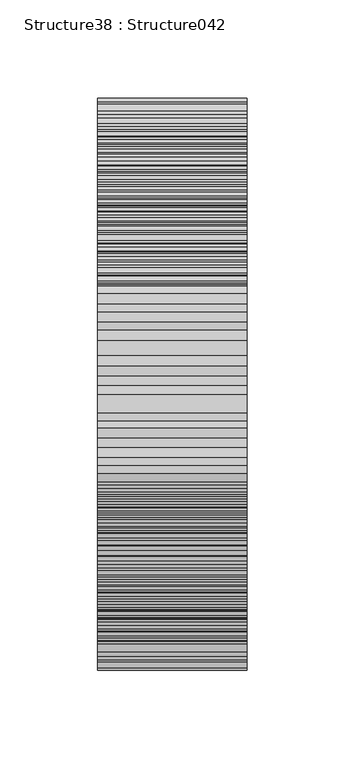
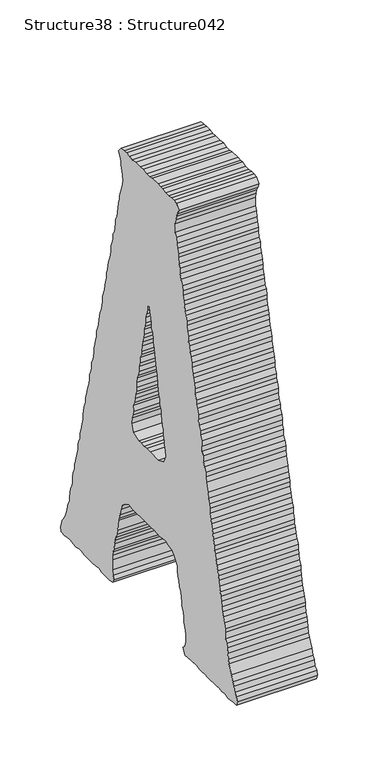
"""IFC4 building model written with IfcOpenShell, lengths in millimetres: proxy geometry, Structure38 : Structure042."""

from ifc_helpers import new_model, si_unit, frame, origin, place, context, project, spatial, polyline, outline, extrude, source, transform, mapped, element, save


def structure38_structure042_37ec2216(model_context):
    return source(origin(), model_context, "Body", "SweptSolid", [
        extrude(outline(polyline([(257160.5137356, 3818.8310229), (257162.8548535, 3824.1149855), (257163.4565802, 3828.2163546), (257164.0358425, 3833.4730389), (257165.7736291, 3838.1761347), (257166.3753558, 3841.6741725), (257168.1356069, 3846.9757858), (257168.1356069, 3851.6612309), (257169.8974627, 3856.9179152), (257171.0784516, 3861.0192843), (257172.236976, 3866.3032469), (257173.3955005, 3870.4030114), (257173.9747627, 3875.0772243), (257175.7366184, 3878.5784713), (257176.3383451, 3884.4609514), (257176.3383451, 3888.5623205), (257177.519334, 3893.822214), (257179.2795852, 3896.763454), (257180.4156451, 3902.6314927), (257181.5966341, 3906.1487857), (257182.777623, 3910.8310217), (257182.777623, 3915.5068392), (257183.9602165, 3919.6066036), (257185.7204676, 3924.8905662), (257187.4582543, 3929.5904528), (257187.4582543, 3934.8503464), (257189.2185054, 3938.3499888), (257190.3994943, 3944.235678), (257190.3994943, 3947.7337158), (257192.1613501, 3952.435207), (257192.7406123, 3957.1190475), (257193.9216012, 3962.3757319), (257195.6593879, 3966.5043792), (257195.6593879, 3974.7055128), (257194.5008634, 3979.3781211), (257193.342339, 3984.0635662), (257191.5596234, 3987.5792547), (257189.2185054, 3992.2614906), (257193.342339, 3996.9645864), (257197.419639, 3997.5486624), (257201.5434725, 3997.5486624), (257206.8033661, 3996.390138), (257211.4823928, 3996.390138), (257216.7647508, 3997.5486624), (257220.285253, 3996.9645864), (257224.3866221, 3997.5486624), (257233.7462802, 3997.5486624), (257238.4493759, 3996.390138), (257243.1300073, 3996.390138), (257248.3882962, 3997.5486624), (257253.6931186, 3996.9645864), (257261.2925255, 3996.9645864), (257266.5748835, 3996.390138), (257270.6521836, 3997.5486624), (257275.957006, 3997.5486624), (257280.0359107, 3996.9645864), (257285.2941996, 3996.390138), (257288.8387709, 3991.6806238), (257286.4751885, 3987.5792547), (257285.2941996, 3983.4794902), (257284.7374018, 3979.9621971), (257283.5564129, 3974.7055128), (257281.7961618, 3965.8930249), (257282.9771507, 3961.794865), (257284.1581396, 3956.5349715), (257287.657782, 3947.1496398), (257287.657782, 3944.235678), (257288.8387709, 3938.9517154), (257289.9972954, 3934.2758979), (257290.599022, 3928.9919353), (257291.780011, 3924.2888396), (257294.0970598, 3919.6066036), (257294.0970598, 3916.0909152), (257294.6779267, 3910.8310217), (257295.8589156, 3906.1487857), (257298.2208934, 3902.6314927), (257298.2208934, 3897.3475301), (257299.9586801, 3892.6636896), (257301.1172045, 3888.5623205), (257301.1172045, 3883.8881076), (257302.299798, 3878.5784713), (257304.0600492, 3873.9203044), (257305.8203003, 3869.8189354), (257306.422027, 3866.3032469), (257307.0012892, 3861.0192843), (257308.7390759, 3856.9179152), (257308.7390759, 3851.6612309), (257310.5009316, 3846.9757858), (257311.1026583, 3842.8583706), (257312.2611827, 3837.6000817), (257315.1799583, 3829.374879), (257315.1799583, 3824.1149855), (257316.3609472, 3820.015221), (257317.5435407, 3815.3313805), (257319.8830541, 3810.0474179), (257320.4847808, 3806.5317294), (257321.6433052, 3801.8462843), (257322.2450319, 3797.1463977), (257323.9828186, 3791.8865042), (257325.1654121, 3788.3611881), (257325.1654121, 3783.0868532), (257326.9256632, 3777.8285642), (257327.5049254, 3774.3032481), (257329.2651766, 3769.0176809), (257329.8669033, 3764.3611187), (257330.423701, 3759.6596275), (257331.6046899, 3756.1423345), (257333.3665457, 3751.4424479), (257333.9458079, 3745.6000829), (257335.1267968, 3740.9162424), (257336.8870479, 3737.9750024), (257336.8870479, 3732.7167134), (257338.0455724, 3727.4311462), (257339.8074281, 3723.3313817), (257340.988417, 3718.0554422), (257342.1469415, 3714.5301261), (257343.3279304, 3710.4560353), (257343.3279304, 3705.7545441), (257345.6449793, 3699.8881101), (257346.8275728, 3695.2122926), (257347.4292995, 3691.0868544), (257347.4292995, 3686.4030139), (257348.5878239, 3682.8857208), (257350.348075, 3677.0449605), (257350.9498017, 3673.5276674), (257352.6875884, 3668.8261762), (257352.6875884, 3663.5598643), (257355.0287064, 3659.4584952), (257356.2096953, 3655.3587307), (257356.2096953, 3650.6845178), (257357.3906842, 3645.4262289), (257359.1509353, 3640.114988), (257360.3094598, 3636.0408972), (257361.4695888, 3632.5155811), (257362.0713155, 3627.2396415), (257363.8315666, 3622.555801), (257365.0125555, 3617.2718384), (257365.0125555, 3612.5976255), (257365.5918178, 3608.4705827), (257367.9313311, 3604.3964919), (257369.0914602, 3599.1125293), (257370.2724491, 3594.4286888), (257370.2724491, 3590.3289243), (257372.0327002, 3586.2115092), (257374.9514758, 3576.2693797), (257376.7133315, 3572.1423369), (257378.4735826, 3568.6426945), (257381.9940849, 3563.366755), (257383.1526094, 3560.441561), (257384.9144651, 3555.1848766), (257383.7334762, 3551.0658569), (257377.8943204, 3550.4833855), (257374.394678, 3551.0658569), (257369.0914602, 3551.6675836), (257364.4108288, 3550.4833855), (257359.1509353, 3550.4833855), (257354.4494441, 3551.6675836), (257350.348075, 3551.6675836), (257345.6449793, 3551.0658569), (257341.5676792, 3551.0658569), (257335.706059, 3550.4833855), (257331.6046899, 3550.4833855), (257326.9256632, 3551.0658569), (257321.6433052, 3551.6675836), (257317.5435407, 3550.4833855), (257304.0600492, 3550.4833855), (257298.8001556, 3551.6675836), (257296.4381778, 3555.7416744), (257298.2208934, 3559.2669905), (257299.3794178, 3563.9412034), (257299.3794178, 3573.9266571), (257299.3794178, 3578.6104977), (257298.2208934, 3582.7102621), (257296.4381778, 3586.2115092), (257295.8589156, 3592.0955938), (257294.6779267, 3596.1953583), (257292.9160709, 3600.2967274), (257291.780011, 3604.3964919), (257290.599022, 3609.0723094), (257289.4180331, 3619.6145609), (257288.2370442, 3622.555801), (257286.4751885, 3627.2396415), (257285.2941996, 3633.0980525), (257282.3978885, 3638.9580681), (257278.2740549, 3642.4833842), (257271.8331725, 3645.9830266), (257267.1541458, 3644.8245022), (257257.7720233, 3644.8245022), (257251.9104031, 3645.4262289), (257239.6303648, 3645.4262289), (257234.3255424, 3644.8245022), (257230.2482424, 3645.9830266), (257225.5451466, 3645.4262289), (257220.8661199, 3644.8245022), (257216.7647508, 3645.4262289), (257210.9031306, 3645.9830266), (257207.3826283, 3644.8245022), (257200.3624836, 3643.0578326), (257196.8403768, 3639.5405396), (257192.1613501, 3633.0980525), (257192.1613501, 3627.8397636), (257190.9803611, 3622.555801), (257189.2185054, 3619.6145609), (257188.6392432, 3613.772196), (257186.2997298, 3610.2292293), (257185.1187409, 3604.9709403), (257184.5394787, 3601.4536473), (257184.5394787, 3596.7698067), (257182.1983607, 3592.0955938), (257181.5966341, 3587.3860796), (257181.0173718, 3582.7102621), (257179.2795852, 3578.6104977), (257177.519334, 3572.7440636), (257178.0985963, 3565.1254015), (257179.8588474, 3559.2669905), (257182.777623, 3556.3417965), (257179.2795852, 3550.4833855), (257173.9747627, 3551.0658569), (257169.295736, 3551.6675836), (257159.9344734, 3551.6675836), (257155.2554467, 3551.0658569), (257150.5523509, 3551.0658569), (257146.4525864, 3551.6675836), (257142.3287528, 3551.0658569), (257136.4895971, 3551.0658569), (257132.9915593, 3551.6675836), (257127.1299391, 3551.0658569), (257123.6078322, 3551.6675836), (257118.9288055, 3550.4833855), (257113.623983, 3551.6675836), (257108.3640895, 3550.4833855), (257104.264325, 3551.0658569), (257099.5612292, 3551.6675836), (257094.904667, 3551.6675836), (257093.1203468, 3556.3417965), (257094.3029403, 3560.441561), (257097.2441803, 3563.366755), (257098.4027048, 3568.6426945), (257100.1629559, 3572.1423369), (257102.5040739, 3577.4535778), (257106.6038383, 3586.2115092), (257107.7848273, 3589.7544759), (257108.3640895, 3595.5872132), (257109.546683, 3600.2967274), (257110.7052074, 3604.3964919), (257112.4654586, 3607.8961343), (257113.0447208, 3613.772196), (257113.0447208, 3617.2718384), (257114.2257097, 3622.555801), (257115.9859608, 3627.8397636), (257117.7478166, 3631.915459), (257118.9288055, 3636.0408972), (257119.5080677, 3641.2991861), (257120.0648655, 3645.9830266), (257120.6665921, 3650.1004418), (257123.0061055, 3654.1841602), (257123.6078322, 3660.0682449), (257124.188699, 3664.1423357), (257124.7679612, 3668.8261762), (257126.5282124, 3672.9435914), (257128.2884635, 3677.6274319), (257129.4469879, 3682.8857208), (257130.6279769, 3685.8285655), (257130.6279769, 3690.512406), (257132.3898326, 3695.786741), (257132.9915593, 3701.0723082), (257134.1500837, 3704.5879966), (257135.8878704, 3709.2718371), (257136.4895971, 3713.3555556), (257138.2498482, 3718.6571688), (257138.2498482, 3723.3313817), (257139.4324417, 3727.4311462), (257140.5909662, 3732.1149867), (257141.7719551, 3737.400554), (257144.1114684, 3746.1745313), (257145.2699929, 3750.8583719), (257145.2699929, 3755.559863), (257147.0318486, 3759.6596275), (257148.7920997, 3763.759392), (257148.7920997, 3769.6274306), (257151.1316131, 3773.11905), (257151.1316131, 3777.8285642), (257151.7108753, 3783.0868532), (257154.0744577, 3787.7867397), (257154.0744577, 3791.8865042), (257156.4139711, 3795.960595), (257157.0156978, 3801.8462843), (257157.0156978, 3805.9476534), (257159.3327467, 3811.2043377), (257160.5137356, 3814.7296538), (257160.5137356, 3818.8310229)]), holes=[polyline([(257223.2056332, 3720.4158154), (257236.6891248, 3720.4158154), (257241.9474137, 3720.9726131), (257247.2297717, 3719.8140887), (257251.3311408, 3720.9726131), (257255.4309053, 3720.4158154), (257264.2113011, 3723.3313817), (257267.1541458, 3730.9323932), (257265.9731569, 3736.7988273), (257264.8130278, 3740.9162424), (257263.6320389, 3744.9999608), (257264.2113011, 3750.8583719), (257261.8942522, 3754.9854146), (257261.2925255, 3759.6596275), (257260.7132633, 3763.759392), (257258.9530122, 3767.8607611), (257258.3512855, 3772.5606477), (257258.3512855, 3777.2444882), (257257.7720233, 3782.5027771), (257256.0101675, 3786.0280932), (257254.8516431, 3790.7039107), (257254.8516431, 3795.4037973), (257252.5121297, 3800.6717138), (257252.5121297, 3805.9476534), (257250.7518786, 3810.0474179), (257250.1501519, 3813.5743386), (257249.5692851, 3819.4150989), (257248.3882962, 3824.1149855), (257247.2297717, 3828.790803), (257246.6505095, 3832.8921721), (257246.6505095, 3837.6000817), (257244.3109962, 3842.2758992), (257243.7092695, 3846.3772683), (257243.7092695, 3851.6612309), (257241.9474137, 3856.3161885), (257240.7664248, 3860.4432313), (257240.7664248, 3864.5446004), (257239.0286382, 3865.1190488), (257237.8701137, 3860.4432313), (257236.0873981, 3855.7353217), (257235.5081359, 3851.0595042), (257235.5081359, 3845.8012153), (257233.1670179, 3842.2758992), (257232.5652913, 3836.9919366), (257232.5652913, 3833.4730389), (257230.2482424, 3828.790803), (257229.6465157, 3822.932392), (257229.0672535, 3818.8310229), (257227.8862645, 3814.7296538), (257227.3053977, 3810.0474179), (257225.5451466, 3804.7730829), (257224.9434199, 3795.4037973), (257223.8073599, 3790.7039107), (257223.2056332, 3786.0280932), (257221.4453821, 3783.0868532), (257221.4453821, 3777.8285642), (257219.1042641, 3773.11905), (257219.1042641, 3768.4432325), (257217.9232752, 3764.3611187), (257217.344013, 3759.0595054), (257215.6062263, 3755.559863), (257215.6062263, 3750.3015741), (257213.8235107, 3744.9999608), (257213.8235107, 3741.5003184), (257212.6633817, 3736.7988273), (257211.4823928, 3730.9323932), (257215.0044997, 3723.9154578), (257223.2056332, 3720.4158154)])]), frame((-38594.2176606, 0.0, 0.0), z_axis=(1.0, 0.0, 0.0), x_axis=(0.0, 1.0, 0.0)), (0.0, 0.0, 1.0), 76.2),
    ])


if __name__ == "__main__":
    model = new_model("IFC4")
    model_context = context("Model", 3, world=origin())
    ifc_project = project(units=[si_unit("LENGTHUNIT", "METRE", prefix="MILLI")], contexts=[model_context])
    site = spatial("IfcSite", under=ifc_project)
    building = spatial("IfcBuilding", under=site)
    placement = place(None, origin())
    structure38_structure042_shape = structure38_structure042_37ec2216(model_context)
    element("IfcBuildingElementProxy", 1, Name="Structure38 : Structure042", ObjectType="Structure38 : Structure042", at=placement, inside=building, context=model_context, shape_type="MappedRepresentation", body=[
        mapped(structure38_structure042_shape, transform((0.0, 0.0, 0.0), x_axis=(1.0, 0.0, 0.0), y_axis=(0.0, 1.0, 0.0), z_axis=(0.0, 0.0, 1.0))),
    ])
    save(model, "model.ifc")

# Revit data of these elements
# Type "Structure38 : Structure042"
#   NameOverride = "Structure042"
# Element 1 (IfcBuildingElementProxy, "Structure38 : Structure042")
#   Materials on its faces: "BRUSHED ALUM. LETTERING"
# Materials
#   "BRUSHED ALUM. LETTERING": class "Unassigned", colour RGB 169 181 186, transparency 0, Cost = 0
